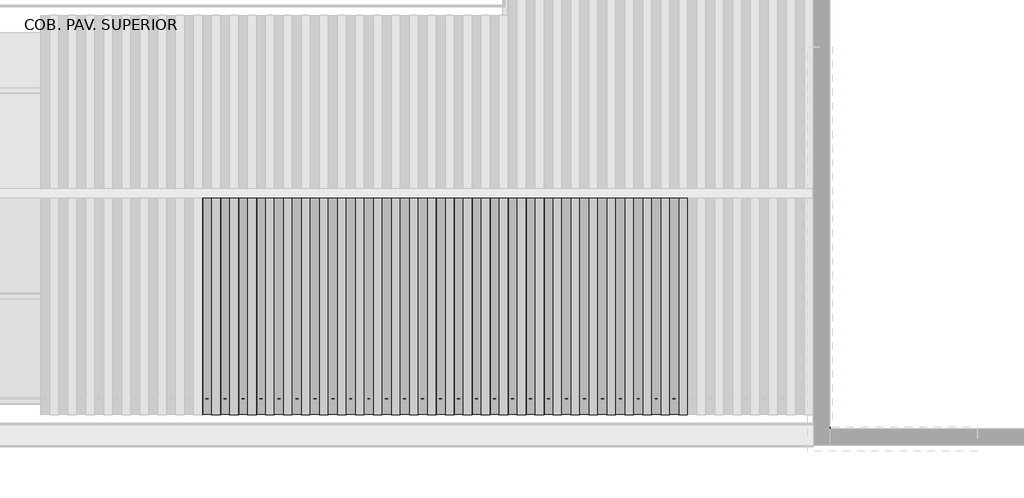
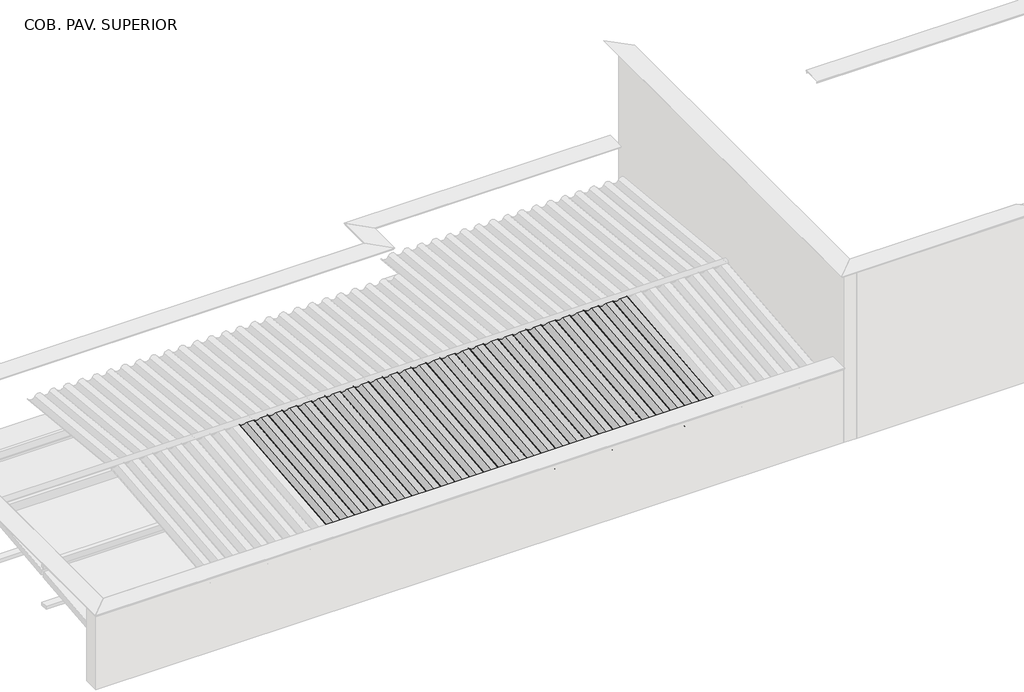
# One storey, part 2 of 7: 35 beams, 8 columns.
"""IFC4 building model written with IfcOpenShell, lengths in millimetres."""

import ifcopenshell
import ifcopenshell.guid

model = None  # the IFC model being written
_history = None  # IfcOwnerHistory: only IFC2X3 demands one
_inside = {}  # id of a spatial element -> (the spatial element, [elements in it])
_under = {}  # id of a project, library or spatial element -> (it, [spatial elements below it])
_declared = {}  # id of a project -> (the project, [libraries it declares])
_typed = {}  # id of a type object -> (the type object, [elements of that type])
_made_of = {}  # id of a material, layer set ... -> (it, [elements and type objects made of it])


def new_model(schema):
    """Start an empty IFC model of exactly this schema.

    Asked for "IFC4X3", IfcOpenShell would pick the latest addendum, in which some entities
    have other attributes; the version numbers below select the first issue.
    IFC2X3 requires an IfcOwnerHistory on every rooted entity: one is made here for all.
    """
    global model, _history
    if schema == "IFC4X3":
        model = ifcopenshell.file(schema_version=(4, 3, 0, 0))
    else:
        model = ifcopenshell.file(schema=schema)
    _inside.clear()
    _under.clear()
    _declared.clear()
    _typed.clear()
    _made_of.clear()
    _history = None
    if model.schema == "IFC2X3":
        org = make("IfcOrganization", Name="unknown")
        user = make(
            "IfcPersonAndOrganization",
            ThePerson=make("IfcPerson", FamilyName="unknown"),
            TheOrganization=org,
        )
        app = make(
            "IfcApplication",
            ApplicationDeveloper=org,
            Version="unknown",
            ApplicationFullName="unknown",
            ApplicationIdentifier="unknown",
        )
        _history = make(
            "IfcOwnerHistory",
            OwningUser=user,
            OwningApplication=app,
            ChangeAction="ADDED",
            CreationDate=0,
        )
    return model


def make(cls, **values):
    """One entity of the class cls with the attributes given. An attribute that is None is left unset."""
    return model.create_entity(
        cls, **{name: value for name, value in values.items() if value is not None}
    )


def rooted(cls, **values):
    """An entity with a GlobalId (a new one), such as an element, a storey or a relation."""
    return make(cls, GlobalId=ifcopenshell.guid.new(), OwnerHistory=_history, **values)


def si_unit(unit_type, name, prefix=None):
    """IfcSIUnit, for example si_unit("LENGTHUNIT", "METRE", prefix="MILLI")."""
    return make("IfcSIUnit", UnitType=unit_type, Prefix=prefix, Name=name)


def assignment(units):
    """IfcUnitAssignment: the units of a project."""
    return None if units is None else make("IfcUnitAssignment", Units=units)


def point(xyz):
    """IfcCartesianPoint."""
    return None if xyz is None else make("IfcCartesianPoint", Coordinates=xyz)


def direction(xyz):
    """IfcDirection."""
    return None if xyz is None else make("IfcDirection", DirectionRatios=xyz)


def frame(location, z_axis=None, x_axis=None):
    """IfcAxis2Placement3D, a coordinate frame: its origin and axes. An axis left out is left unset."""
    return make(
        "IfcAxis2Placement3D",
        Location=point(location),
        Axis=direction(z_axis),
        RefDirection=direction(x_axis),
    )


def frame_2d(location, x_axis=None):
    """IfcAxis2Placement2D, a coordinate frame in the plane: its origin and x axis."""
    return make(
        "IfcAxis2Placement2D", Location=point(location), RefDirection=direction(x_axis)
    )


def origin():
    """The frame at (0, 0, 0) with its axes left unset."""
    return frame((0.0, 0.0, 0.0))


def place(relative_to, where):
    """IfcLocalPlacement: puts the frame where relative to a parent placement (None: the world)."""
    return make(
        "IfcLocalPlacement", PlacementRelTo=relative_to, RelativePlacement=where
    )


def context(
    kind, dimensions, precision=None, world=None, true_north=None, identifier=None
):
    """IfcGeometricRepresentationContext, for example the 3D "Model" context."""
    return make(
        "IfcGeometricRepresentationContext",
        ContextIdentifier=identifier,
        ContextType=kind,
        CoordinateSpaceDimension=dimensions,
        Precision=precision,
        WorldCoordinateSystem=world,
        TrueNorth=true_north,
    )


def project(units=None, contexts=None):
    """IfcProject with its units and contexts."""
    return rooted(
        "IfcProject",
        Name="project",
        RepresentationContexts=contexts,
        UnitsInContext=assignment(units),
    )


def spatial(cls, under=None, at=None, **own):
    """A site, building, storey or space (cls), placed at a placement, below another one or the project."""
    s = rooted(cls, ObjectPlacement=at, **own)
    if under is not None:
        _under.setdefault(under.id(), (under, []))[1].append(s)
    return s


def polyline(points):
    """IfcPolyline through the points."""
    return make("IfcPolyline", Points=[point(p) for p in points])


def circle_curve(where, radius):
    """IfcCircle in the frame where."""
    return make("IfcCircle", Position=where, Radius=radius)


def trimmed(basis, trim1, trim2, sense, master):
    """IfcTrimmedCurve: the piece of a basis curve between two trims."""
    return make(
        "IfcTrimmedCurve",
        BasisCurve=basis,
        Trim1=trim1,
        Trim2=trim2,
        SenseAgreement=sense,
        MasterRepresentation=master,
    )


def segment(curve, same_sense, transition):
    """IfcCompositeCurveSegment."""
    return make(
        "IfcCompositeCurveSegment",
        Transition=transition,
        SameSense=same_sense,
        ParentCurve=curve,
    )


def composite_curve(segments, self_intersect=None):
    """IfcCompositeCurve: segments joined end to end."""
    return make("IfcCompositeCurve", Segments=segments, SelfIntersect=self_intersect)


def outline(outer, holes=None, kind="AREA"):
    """IfcArbitraryClosedProfileDef: a profile drawn as a closed curve; with holes, ...WithVoids."""
    if holes is None:
        return make("IfcArbitraryClosedProfileDef", ProfileType=kind, OuterCurve=outer)
    return make(
        "IfcArbitraryProfileDefWithVoids",
        ProfileType=kind,
        OuterCurve=outer,
        InnerCurves=holes,
    )


def extrude(swept, where, along, depth):
    """IfcExtrudedAreaSolid: the profile swept, set in the frame where, extruded along a direction by depth."""
    return make(
        "IfcExtrudedAreaSolid",
        SweptArea=swept,
        Position=where,
        ExtrudedDirection=direction(along),
        Depth=depth,
    )


def faces_of(points, faces, orient=None, outer=None):
    """IfcFace entities. A face is a list of loops; a loop is a list of indices into points, from 0.

    orient and outer hold one flag for each loop. By default every Orientation is true, the
    first loop of a face is its IfcFaceOuterBound and the others are IfcFaceBound.
    """
    made = []
    for i, loops in enumerate(faces):
        bounds = []
        for j, loop in enumerate(loops):
            is_outer = j == 0 if outer is None else outer[i][j]
            bounds.append(
                make(
                    "IfcFaceOuterBound" if is_outer else "IfcFaceBound",
                    Bound=make("IfcPolyLoop", Polygon=[points[k] for k in loop]),
                    Orientation=True if orient is None else orient[i][j],
                )
            )
        made.append(make("IfcFace", Bounds=bounds))
    return made


def faceted_brep(points, faces, orient=None, outer=None, voids=None):
    """IfcFacetedBrep: a solid bounded by flat faces; with voids (closed shells), ...WithVoids."""
    shared = [point(p) for p in points]
    hull = make("IfcClosedShell", CfsFaces=faces_of(shared, faces, orient, outer))
    if voids is None:
        return make("IfcFacetedBrep", Outer=hull)
    return make(
        "IfcFacetedBrepWithVoids",
        Outer=hull,
        Voids=[
            make(cls, CfsFaces=faces_of(shared, fs, o, b)) for cls, fs, o, b in voids
        ],
    )


def shape(context_of_items, identifier, shape_type, items):
    """IfcShapeRepresentation: the items that make up one representation, for example the "Body"."""
    return make(
        "IfcShapeRepresentation",
        ContextOfItems=context_of_items,
        RepresentationIdentifier=identifier,
        RepresentationType=shape_type,
        Items=items,
    )


def source(mapping_origin, context_of_items, identifier, shape_type, items):
    """IfcRepresentationMap: a shape defined once, which mapped items show again and again."""
    return make(
        "IfcRepresentationMap",
        MappingOrigin=mapping_origin,
        MappedRepresentation=shape(context_of_items, identifier, shape_type, items),
    )


def transform(
    local_origin,
    x_axis=None,
    y_axis=None,
    z_axis=None,
    scale=None,
    scale2=None,
    scale3=None,
    uniform=True,
):
    """IfcCartesianTransformationOperator3D, or its non-uniform kind. x_axis, y_axis, z_axis: its Axis1, 2, 3."""
    if uniform:
        return make(
            "IfcCartesianTransformationOperator3D",
            Axis1=direction(x_axis),
            Axis2=direction(y_axis),
            LocalOrigin=point(local_origin),
            Scale=scale,
            Axis3=direction(z_axis),
        )
    return make(
        "IfcCartesianTransformationOperator3DnonUniform",
        Axis1=direction(x_axis),
        Axis2=direction(y_axis),
        LocalOrigin=point(local_origin),
        Scale=scale,
        Axis3=direction(z_axis),
        Scale2=scale2,
        Scale3=scale3,
    )


def mapped(mapping_source, mapping_target):
    """IfcMappedItem: shows the shape of a source again, moved by a transform."""
    return make(
        "IfcMappedItem", MappingSource=mapping_source, MappingTarget=mapping_target
    )


def made_of(thing, what):
    """Note that an element or type object is made of a material, layer set ...; save() writes the relation."""
    if what is not None:
        _made_of.setdefault(what.id(), (what, []))[1].append(thing)
    return thing


def element(
    cls,
    number,
    at=None,
    inside=None,
    cuts=None,
    type_object=None,
    material=None,
    context=None,
    identifier="Body",
    shape_type=None,
    held_by="IfcProductDefinitionShape",
    body=None,
    shapes=None,
    **own,
):
    """One element of the class cls, such as IfcWall. Its Tag is "e" and its number.

    at: its placement. inside: the storey or other place that contains it. cuts: it is an
    opening in that element (IfcRelVoidsElement). A single representation is given by context,
    identifier, shape_type and body (its items); several are given by shapes. held_by: the class
    of the entity that holds the representations. save() writes the other relations.
    """
    e = rooted(cls, Tag="e%d" % number, ObjectPlacement=at, **own)
    if body is not None:
        shapes = [shape(context, identifier, shape_type, body)]
    if shapes is not None:
        e.Representation = make(held_by, Representations=shapes)
    if inside is not None:
        _inside.setdefault(inside.id(), (inside, []))[1].append(e)
    if cuts is not None:
        rooted(
            "IfcRelVoidsElement", RelatingBuildingElement=cuts, RelatedOpeningElement=e
        )
    if type_object is not None:
        _typed.setdefault(type_object.id(), (type_object, []))[1].append(e)
    return made_of(e, material)


def aggregate(whole, parts):
    """IfcRelAggregates: a whole, such as a stair, and the parts it consists of."""
    return rooted("IfcRelAggregates", RelatingObject=whole, RelatedObjects=parts)


def save(model, path):
    """Write the relations noted so far, then the file.

    IfcRelAggregates (storeys below a building ...), IfcRelContainedInSpatialStructure (elements
    in a storey), IfcRelDefinesByType, IfcRelAssociatesMaterial and IfcRelDeclares: one each for
    every whole, place, type object, material and project.
    """
    for whole, parts in _under.values():
        aggregate(whole, parts)
    for where, things in _inside.values():
        rooted(
            "IfcRelContainedInSpatialStructure",
            RelatedElements=things,
            RelatingStructure=where,
        )
    for kind, things in _typed.values():
        rooted("IfcRelDefinesByType", RelatedObjects=things, RelatingType=kind)
    for what, things in _made_of.values():
        rooted("IfcRelAssociatesMaterial", RelatedObjects=things, RelatingMaterial=what)
    for by, libraries in _declared.values():
        rooted("IfcRelDeclares", RelatingContext=by, RelatedDefinitions=libraries)
    model.write(path)


def column_4db371bd(model_context):
    return source(origin(), model_context, "Body", "SweptSolid", [
        extrude(outline(polyline([(30.0, 80.0), (30.0, -80.0), (-30.0, -80.0), (-30.0, 80.0), (30.0, 80.0)])), frame((0.0, 0.0, 6710.0), z_axis=(0.0, 0.0, 1.0), x_axis=(1.0, 0.0, 0.0)), (0.0, 0.0, 1.0), 660.0),
    ])


def column_e8b88e91(model_context):
    return source(origin(), model_context, "Body", "SweptSolid", [
        extrude(outline(polyline([(30.0, 80.0), (30.0, -80.0), (-30.0, -80.0), (-30.0, 80.0), (30.0, 80.0)])), frame((0.0, 0.0, 6710.0), z_axis=(0.0, 0.0, 1.0), x_axis=(1.0, 0.0, 0.0)), (0.0, 0.0, 1.0), 515.0),
    ])


model = new_model("IFC4")

# Units and contexts
model_context = context("Model", 3, world=origin())
ifc_project = project(units=[si_unit("LENGTHUNIT", "METRE", prefix="MILLI")], contexts=[model_context])

# Site, building, storey
site = spatial("IfcSite", under=ifc_project)
building = spatial("IfcBuilding", under=site)
storey = spatial("IfcBuildingStorey", under=building, Name="COB. PAV. SUPERIOR", Elevation=6650.0)

# Beams
placement = place(None, origin())
element("IfcBeam", 1, ObjectType="Madeira de lei : Berço 6x12cm", at=placement, inside=storey, context=model_context, shape_type="SweptSolid", body=[
    extrude(outline(polyline([(-6679.281307, -9101.268869), (-6679.281307, -9221.268869), (-8679.281307, -9221.268869), (-8679.281307, -9101.268869), (-6679.281307, -9101.268869)])), frame((0.0, 0.0, 6650.0), z_axis=(0.0, 0.0, 1.0), x_axis=(1.0, 0.0, 0.0)), (0.0, 0.0, 1.0), 60.0),
])
element("IfcBeam", 2, ObjectType="Madeira de lei : Berço 6x12cm", at=placement, inside=storey, context=model_context, shape_type="SweptSolid", body=[
    extrude(outline(polyline([(-6679.281307, -10521.818869), (-6679.281307, -10641.818869), (-8679.281307, -10641.818869), (-8679.281307, -10521.818869), (-6679.281307, -10521.818869)])), frame((0.0, 0.0, 6650.0), z_axis=(0.0, 0.0, 1.0), x_axis=(1.0, 0.0, 0.0)), (0.0, 0.0, 1.0), 60.0),
])
element("IfcBeam", 3, ObjectType="Madeira de lei : Berço 6x12cm", at=placement, inside=storey, context=model_context, shape_type="SweptSolid", body=[
    extrude(outline(polyline([(-4679.281307, -9101.268869), (-4679.281307, -9221.268869), (-6679.281307, -9221.268869), (-6679.281307, -9101.268869), (-4679.281307, -9101.268869)])), frame((0.0, 0.0, 6650.0), z_axis=(0.0, 0.0, 1.0), x_axis=(1.0, 0.0, 0.0)), (0.0, 0.0, 1.0), 60.0),
])
element("IfcBeam", 4, ObjectType="Madeira de lei : Berço 6x12cm", at=placement, inside=storey, context=model_context, shape_type="SweptSolid", body=[
    extrude(outline(polyline([(-4679.281307, -10521.818869), (-4679.281307, -10641.818869), (-6679.281307, -10641.818869), (-6679.281307, -10521.818869), (-4679.281307, -10521.818869)])), frame((0.0, 0.0, 6650.0), z_axis=(0.0, 0.0, 1.0), x_axis=(1.0, 0.0, 0.0)), (0.0, 0.0, 1.0), 60.0),
])
element("IfcBeam", 5, ObjectType="Madeira de lei : Berço 6x12cm", at=placement, inside=storey, context=model_context, shape_type="SweptSolid", body=[
    extrude(outline(polyline([(-2679.281307, -9101.268869), (-2679.281307, -9221.268869), (-4679.281307, -9221.268869), (-4679.281307, -9101.268869), (-2679.281307, -9101.268869)])), frame((0.0, 0.0, 6650.0), z_axis=(0.0, 0.0, 1.0), x_axis=(1.0, 0.0, 0.0)), (0.0, 0.0, 1.0), 60.0),
])
element("IfcBeam", 6, ObjectType="Madeira de lei : Berço 6x12cm", at=placement, inside=storey, context=model_context, shape_type="SweptSolid", body=[
    extrude(outline(polyline([(-2679.281307, -10521.818869), (-2679.281307, -10641.818869), (-4679.281307, -10641.818869), (-4679.281307, -10521.818869), (-2679.281307, -10521.818869)])), frame((0.0, 0.0, 6650.0), z_axis=(0.0, 0.0, 1.0), x_axis=(1.0, 0.0, 0.0)), (0.0, 0.0, 1.0), 60.0),
])
element("IfcBeam", 7, ObjectType="Madeira de lei : Berço 6x12cm", at=placement, inside=storey, context=model_context, shape_type="SweptSolid", body=[
    extrude(outline(polyline([(-679.281307, -10521.818869), (-679.281307, -10641.818869), (-2679.281307, -10641.818869), (-2679.281307, -10521.818869), (-679.281307, -10521.818869)])), frame((0.0, 0.0, 6650.0), z_axis=(0.0, 0.0, 1.0), x_axis=(1.0, 0.0, 0.0)), (0.0, 0.0, 1.0), 60.0),
])
element("IfcBeam", 8, ObjectType="Madeira de lei : Berço 6x12cm", at=placement, inside=storey, context=model_context, shape_type="SweptSolid", body=[
    extrude(outline(polyline([(-239.281307, -10521.818869), (-239.281307, -10641.818869), (-679.281307, -10641.818869), (-679.281307, -10521.818869), (-239.281307, -10521.818869)])), frame((0.0, 0.0, 6650.0), z_axis=(0.0, 0.0, 1.0), x_axis=(1.0, 0.0, 0.0)), (0.0, 0.0, 1.0), 60.0),
])
element("IfcBeam", 9, ObjectType="Telha Ondulada : Fibrocimento", at=placement, inside=storey, context=model_context, shape_type="SweptSolid", body=[
    extrude(outline(composite_curve([segment(trimmed(circle_curve(frame_2d((0.0, 66.7939461)), 66.7939461), [point((29.3501489, 6.7939461))], [point((29.3501489, 126.7939461))], True, "CARTESIAN"), True, "CONTINUOUS"), segment(polyline([(29.3501489, 126.7939461), (31.5472154, 131.2853711)]), True, "CONTINUOUS"), segment(trimmed(circle_curve(frame_2d((0.0, 66.7939461)), 71.7939461), [point((31.5472154, 131.2853711))], [point((31.5472154, 2.3025211))], False, "CARTESIAN"), True, "CONTINUOUS"), segment(trimmed(circle_curve(frame_2d((58.7002978, -53.2060539)), 61.7939461), [point((31.5472154, 2.3025211))], [point((31.5472154, -108.7146289))], True, "CARTESIAN"), True, "CONTINUOUS"), segment(polyline([(31.5472154, -108.7146289), (29.3501489, -113.2060539)]), True, "CONTINUOUS"), segment(trimmed(circle_curve(frame_2d((58.7002978, -53.2060539)), 66.7939461), [point((29.3501489, -113.2060539))], [point((29.3501489, 6.7939461))], False, "CARTESIAN"), True, "CONTINUOUS")], self_intersect=False)), frame((-8428.8843743, -10781.9594023, 7394.5315886), z_axis=(0.0, 0.9950371902099894, 0.0995037190209974), x_axis=(0.0, 0.0995037190209974, -0.9950371902099894)), (0.0, 0.0, 1.0), 3017.2295147),
])
element("IfcBeam", 10, ObjectType="Telha Ondulada : Fibrocimento", at=placement, inside=storey, context=model_context, shape_type="SweptSolid", body=[
    extrude(outline(composite_curve([segment(trimmed(circle_curve(frame_2d((0.0, 66.7939461)), 66.7939461), [point((29.3501489, 6.7939461))], [point((29.3501489, 126.7939461))], True, "CARTESIAN"), True, "CONTINUOUS"), segment(polyline([(29.3501489, 126.7939461), (31.5472154, 131.2853711)]), True, "CONTINUOUS"), segment(trimmed(circle_curve(frame_2d((0.0, 66.7939461)), 71.7939461), [point((31.5472154, 131.2853711))], [point((31.5472154, 2.3025211))], False, "CARTESIAN"), True, "CONTINUOUS"), segment(trimmed(circle_curve(frame_2d((58.7002978, -53.2060539)), 61.7939461), [point((31.5472154, 2.3025211))], [point((31.5472154, -108.7146289))], True, "CARTESIAN"), True, "CONTINUOUS"), segment(polyline([(31.5472154, -108.7146289), (29.3501489, -113.2060539)]), True, "CONTINUOUS"), segment(trimmed(circle_curve(frame_2d((58.7002978, -53.2060539)), 66.7939461), [point((29.3501489, -113.2060539))], [point((29.3501489, 6.7939461))], False, "CARTESIAN"), True, "CONTINUOUS")], self_intersect=False)), frame((-8184.3843743, -10781.9594023, 7394.5315886), z_axis=(0.0, 0.9950371902099894, 0.09950371902099736), x_axis=(0.0, 0.09950371902099736, -0.9950371902099894)), (0.0, 0.0, 1.0), 3017.2295147),
])
element("IfcBeam", 11, ObjectType="Telha Ondulada : Fibrocimento", at=placement, inside=storey, context=model_context, shape_type="SweptSolid", body=[
    extrude(outline(composite_curve([segment(trimmed(circle_curve(frame_2d((0.0, 66.7939461)), 66.7939461), [point((29.3501489, 6.7939461))], [point((29.3501489, 126.7939461))], True, "CARTESIAN"), True, "CONTINUOUS"), segment(polyline([(29.3501489, 126.7939461), (31.5472154, 131.2853711)]), True, "CONTINUOUS"), segment(trimmed(circle_curve(frame_2d((0.0, 66.7939461)), 71.7939461), [point((31.5472154, 131.2853711))], [point((31.5472154, 2.3025211))], False, "CARTESIAN"), True, "CONTINUOUS"), segment(trimmed(circle_curve(frame_2d((58.7002978, -53.2060539)), 61.7939461), [point((31.5472154, 2.3025211))], [point((31.5472154, -108.7146289))], True, "CARTESIAN"), True, "CONTINUOUS"), segment(polyline([(31.5472154, -108.7146289), (29.3501489, -113.2060539)]), True, "CONTINUOUS"), segment(trimmed(circle_curve(frame_2d((58.7002978, -53.2060539)), 66.7939461), [point((29.3501489, -113.2060539))], [point((29.3501489, 6.7939461))], False, "CARTESIAN"), True, "CONTINUOUS")], self_intersect=False)), frame((-7939.8843743, -10781.9594023, 7394.5315886), z_axis=(0.0, 0.9950371902099894, 0.09950371902099743), x_axis=(0.0, 0.09950371902099743, -0.9950371902099894)), (0.0, 0.0, 1.0), 3017.2295147),
])
element("IfcBeam", 12, ObjectType="Telha Ondulada : Fibrocimento", at=placement, inside=storey, context=model_context, shape_type="SweptSolid", body=[
    extrude(outline(composite_curve([segment(trimmed(circle_curve(frame_2d((0.0, 66.7939461)), 66.7939461), [point((29.3501489, 6.7939461))], [point((29.3501489, 126.7939461))], True, "CARTESIAN"), True, "CONTINUOUS"), segment(polyline([(29.3501489, 126.7939461), (31.5472154, 131.2853711)]), True, "CONTINUOUS"), segment(trimmed(circle_curve(frame_2d((0.0, 66.7939461)), 71.7939461), [point((31.5472154, 131.2853711))], [point((31.5472154, 2.3025211))], False, "CARTESIAN"), True, "CONTINUOUS"), segment(trimmed(circle_curve(frame_2d((58.7002978, -53.2060539)), 61.7939461), [point((31.5472154, 2.3025211))], [point((31.5472154, -108.7146289))], True, "CARTESIAN"), True, "CONTINUOUS"), segment(polyline([(31.5472154, -108.7146289), (29.3501489, -113.2060539)]), True, "CONTINUOUS"), segment(trimmed(circle_curve(frame_2d((58.7002978, -53.2060539)), 66.7939461), [point((29.3501489, -113.2060539))], [point((29.3501489, 6.7939461))], False, "CARTESIAN"), True, "CONTINUOUS")], self_intersect=False)), frame((-7695.3843743, -10781.9594023, 7394.5315886), z_axis=(0.0, 0.9950371902099894, 0.09950371902099743), x_axis=(0.0, 0.09950371902099743, -0.9950371902099894)), (0.0, 0.0, 1.0), 3017.2295147),
])
element("IfcBeam", 13, ObjectType="Telha Ondulada : Fibrocimento", at=placement, inside=storey, context=model_context, shape_type="SweptSolid", body=[
    extrude(outline(composite_curve([segment(trimmed(circle_curve(frame_2d((0.0, 66.7939461)), 66.7939461), [point((29.3501489, 6.7939461))], [point((29.3501489, 126.7939461))], True, "CARTESIAN"), True, "CONTINUOUS"), segment(polyline([(29.3501489, 126.7939461), (31.5472154, 131.2853711)]), True, "CONTINUOUS"), segment(trimmed(circle_curve(frame_2d((0.0, 66.7939461)), 71.7939461), [point((31.5472154, 131.2853711))], [point((31.5472154, 2.3025211))], False, "CARTESIAN"), True, "CONTINUOUS"), segment(trimmed(circle_curve(frame_2d((58.7002978, -53.2060539)), 61.7939461), [point((31.5472154, 2.3025211))], [point((31.5472154, -108.7146289))], True, "CARTESIAN"), True, "CONTINUOUS"), segment(polyline([(31.5472154, -108.7146289), (29.3501489, -113.2060539)]), True, "CONTINUOUS"), segment(trimmed(circle_curve(frame_2d((58.7002978, -53.2060539)), 66.7939461), [point((29.3501489, -113.2060539))], [point((29.3501489, 6.7939461))], False, "CARTESIAN"), True, "CONTINUOUS")], self_intersect=False)), frame((-7450.8843743, -10781.9594023, 7394.5315886), z_axis=(0.0, 0.9950371902099894, 0.09950371902099743), x_axis=(0.0, 0.09950371902099743, -0.9950371902099894)), (0.0, 0.0, 1.0), 3017.2295147),
])
element("IfcBeam", 14, ObjectType="Telha Ondulada : Fibrocimento", at=placement, inside=storey, context=model_context, shape_type="SweptSolid", body=[
    extrude(outline(composite_curve([segment(trimmed(circle_curve(frame_2d((0.0, 66.7939461)), 66.7939461), [point((29.3501489, 6.7939461))], [point((29.3501489, 126.7939461))], True, "CARTESIAN"), True, "CONTINUOUS"), segment(polyline([(29.3501489, 126.7939461), (31.5472154, 131.2853711)]), True, "CONTINUOUS"), segment(trimmed(circle_curve(frame_2d((0.0, 66.7939461)), 71.7939461), [point((31.5472154, 131.2853711))], [point((31.5472154, 2.3025211))], False, "CARTESIAN"), True, "CONTINUOUS"), segment(trimmed(circle_curve(frame_2d((58.7002978, -53.2060539)), 61.7939461), [point((31.5472154, 2.3025211))], [point((31.5472154, -108.7146289))], True, "CARTESIAN"), True, "CONTINUOUS"), segment(polyline([(31.5472154, -108.7146289), (29.3501489, -113.2060539)]), True, "CONTINUOUS"), segment(trimmed(circle_curve(frame_2d((58.7002978, -53.2060539)), 66.7939461), [point((29.3501489, -113.2060539))], [point((29.3501489, 6.7939461))], False, "CARTESIAN"), True, "CONTINUOUS")], self_intersect=False)), frame((-7206.3843743, -10781.9594023, 7394.5315886), z_axis=(0.0, 0.9950371902099894, 0.0995037190209974), x_axis=(0.0, 0.0995037190209974, -0.9950371902099894)), (0.0, 0.0, 1.0), 3017.2295147),
])
element("IfcBeam", 15, ObjectType="Telha Ondulada : Fibrocimento", at=placement, inside=storey, context=model_context, shape_type="SweptSolid", body=[
    extrude(outline(composite_curve([segment(trimmed(circle_curve(frame_2d((0.0, 66.7939461)), 66.7939461), [point((29.3501489, 6.7939461))], [point((29.3501489, 126.7939461))], True, "CARTESIAN"), True, "CONTINUOUS"), segment(polyline([(29.3501489, 126.7939461), (31.5472154, 131.2853711)]), True, "CONTINUOUS"), segment(trimmed(circle_curve(frame_2d((0.0, 66.7939461)), 71.7939461), [point((31.5472154, 131.2853711))], [point((31.5472154, 2.3025211))], False, "CARTESIAN"), True, "CONTINUOUS"), segment(trimmed(circle_curve(frame_2d((58.7002978, -53.2060539)), 61.7939461), [point((31.5472154, 2.3025211))], [point((31.5472154, -108.7146289))], True, "CARTESIAN"), True, "CONTINUOUS"), segment(polyline([(31.5472154, -108.7146289), (29.3501489, -113.2060539)]), True, "CONTINUOUS"), segment(trimmed(circle_curve(frame_2d((58.7002978, -53.2060539)), 66.7939461), [point((29.3501489, -113.2060539))], [point((29.3501489, 6.7939461))], False, "CARTESIAN"), True, "CONTINUOUS")], self_intersect=False)), frame((-6961.8843743, -10781.9594023, 7394.5315886), z_axis=(0.0, 0.9950371902099894, 0.0995037190209974), x_axis=(0.0, 0.0995037190209974, -0.9950371902099894)), (0.0, 0.0, 1.0), 3017.2295147),
])
element("IfcBeam", 16, ObjectType="Telha Ondulada : Fibrocimento", at=placement, inside=storey, context=model_context, shape_type="SweptSolid", body=[
    extrude(outline(composite_curve([segment(trimmed(circle_curve(frame_2d((0.0, 66.7939461)), 66.7939461), [point((29.3501489, 6.7939461))], [point((29.3501489, 126.7939461))], True, "CARTESIAN"), True, "CONTINUOUS"), segment(polyline([(29.3501489, 126.7939461), (31.5472154, 131.2853711)]), True, "CONTINUOUS"), segment(trimmed(circle_curve(frame_2d((0.0, 66.7939461)), 71.7939461), [point((31.5472154, 131.2853711))], [point((31.5472154, 2.3025211))], False, "CARTESIAN"), True, "CONTINUOUS"), segment(trimmed(circle_curve(frame_2d((58.7002978, -53.2060539)), 61.7939461), [point((31.5472154, 2.3025211))], [point((31.5472154, -108.7146289))], True, "CARTESIAN"), True, "CONTINUOUS"), segment(polyline([(31.5472154, -108.7146289), (29.3501489, -113.2060539)]), True, "CONTINUOUS"), segment(trimmed(circle_curve(frame_2d((58.7002978, -53.2060539)), 66.7939461), [point((29.3501489, -113.2060539))], [point((29.3501489, 6.7939461))], False, "CARTESIAN"), True, "CONTINUOUS")], self_intersect=False)), frame((-6717.3843743, -10781.9594023, 7394.5315886), z_axis=(0.0, 0.9950371902099894, 0.09950371902099743), x_axis=(0.0, 0.09950371902099743, -0.9950371902099894)), (0.0, 0.0, 1.0), 3017.2295147),
])
element("IfcBeam", 17, ObjectType="Telha Ondulada : Fibrocimento", at=placement, inside=storey, context=model_context, shape_type="SweptSolid", body=[
    extrude(outline(composite_curve([segment(trimmed(circle_curve(frame_2d((0.0, 66.7939461)), 66.7939461), [point((29.3501489, 6.7939461))], [point((29.3501489, 126.7939461))], True, "CARTESIAN"), True, "CONTINUOUS"), segment(polyline([(29.3501489, 126.7939461), (31.5472154, 131.2853711)]), True, "CONTINUOUS"), segment(trimmed(circle_curve(frame_2d((0.0, 66.7939461)), 71.7939461), [point((31.5472154, 131.2853711))], [point((31.5472154, 2.3025211))], False, "CARTESIAN"), True, "CONTINUOUS"), segment(trimmed(circle_curve(frame_2d((58.7002978, -53.2060539)), 61.7939461), [point((31.5472154, 2.3025211))], [point((31.5472154, -108.7146289))], True, "CARTESIAN"), True, "CONTINUOUS"), segment(polyline([(31.5472154, -108.7146289), (29.3501489, -113.2060539)]), True, "CONTINUOUS"), segment(trimmed(circle_curve(frame_2d((58.7002978, -53.2060539)), 66.7939461), [point((29.3501489, -113.2060539))], [point((29.3501489, 6.7939461))], False, "CARTESIAN"), True, "CONTINUOUS")], self_intersect=False)), frame((-6472.8843743, -10781.9594023, 7394.5315886), z_axis=(0.0, 0.9950371902099894, 0.09950371902099743), x_axis=(0.0, 0.09950371902099743, -0.9950371902099894)), (0.0, 0.0, 1.0), 3017.2295147),
])
element("IfcBeam", 18, ObjectType="Telha Ondulada : Fibrocimento", at=placement, inside=storey, context=model_context, shape_type="SweptSolid", body=[
    extrude(outline(composite_curve([segment(trimmed(circle_curve(frame_2d((0.0, 66.7939461)), 66.7939461), [point((29.3501489, 6.7939461))], [point((29.3501489, 126.7939461))], True, "CARTESIAN"), True, "CONTINUOUS"), segment(polyline([(29.3501489, 126.7939461), (31.5472154, 131.2853711)]), True, "CONTINUOUS"), segment(trimmed(circle_curve(frame_2d((0.0, 66.7939461)), 71.7939461), [point((31.5472154, 131.2853711))], [point((31.5472154, 2.3025211))], False, "CARTESIAN"), True, "CONTINUOUS"), segment(trimmed(circle_curve(frame_2d((58.7002978, -53.2060539)), 61.7939461), [point((31.5472154, 2.3025211))], [point((31.5472154, -108.7146289))], True, "CARTESIAN"), True, "CONTINUOUS"), segment(polyline([(31.5472154, -108.7146289), (29.3501489, -113.2060539)]), True, "CONTINUOUS"), segment(trimmed(circle_curve(frame_2d((58.7002978, -53.2060539)), 66.7939461), [point((29.3501489, -113.2060539))], [point((29.3501489, 6.7939461))], False, "CARTESIAN"), True, "CONTINUOUS")], self_intersect=False)), frame((-6228.3843743, -10781.9594023, 7394.5315886), z_axis=(0.0, 0.9950371902099894, 0.09950371902099743), x_axis=(0.0, 0.09950371902099743, -0.9950371902099894)), (0.0, 0.0, 1.0), 3017.2295147),
])
element("IfcBeam", 19, ObjectType="Telha Ondulada : Fibrocimento", at=placement, inside=storey, context=model_context, shape_type="SweptSolid", body=[
    extrude(outline(composite_curve([segment(trimmed(circle_curve(frame_2d((0.0, 66.7939461)), 66.7939461), [point((29.3501489, 6.7939461))], [point((29.3501489, 126.7939461))], True, "CARTESIAN"), True, "CONTINUOUS"), segment(polyline([(29.3501489, 126.7939461), (31.5472154, 131.2853711)]), True, "CONTINUOUS"), segment(trimmed(circle_curve(frame_2d((0.0, 66.7939461)), 71.7939461), [point((31.5472154, 131.2853711))], [point((31.5472154, 2.3025211))], False, "CARTESIAN"), True, "CONTINUOUS"), segment(trimmed(circle_curve(frame_2d((58.7002978, -53.2060539)), 61.7939461), [point((31.5472154, 2.3025211))], [point((31.5472154, -108.7146289))], True, "CARTESIAN"), True, "CONTINUOUS"), segment(polyline([(31.5472154, -108.7146289), (29.3501489, -113.2060539)]), True, "CONTINUOUS"), segment(trimmed(circle_curve(frame_2d((58.7002978, -53.2060539)), 66.7939461), [point((29.3501489, -113.2060539))], [point((29.3501489, 6.7939461))], False, "CARTESIAN"), True, "CONTINUOUS")], self_intersect=False)), frame((-5983.8843743, -10781.9594023, 7394.5315886), z_axis=(0.0, 0.9950371902099894, 0.09950371902099743), x_axis=(0.0, 0.09950371902099743, -0.9950371902099894)), (0.0, 0.0, 1.0), 3017.2295147),
])
element("IfcBeam", 20, ObjectType="Telha Ondulada : Fibrocimento", at=placement, inside=storey, context=model_context, shape_type="SweptSolid", body=[
    extrude(outline(composite_curve([segment(trimmed(circle_curve(frame_2d((0.0, 66.7939461)), 66.7939461), [point((29.3501489, 6.7939461))], [point((29.3501489, 126.7939461))], True, "CARTESIAN"), True, "CONTINUOUS"), segment(polyline([(29.3501489, 126.7939461), (31.5472154, 131.2853711)]), True, "CONTINUOUS"), segment(trimmed(circle_curve(frame_2d((0.0, 66.7939461)), 71.7939461), [point((31.5472154, 131.2853711))], [point((31.5472154, 2.3025211))], False, "CARTESIAN"), True, "CONTINUOUS"), segment(trimmed(circle_curve(frame_2d((58.7002978, -53.2060539)), 61.7939461), [point((31.5472154, 2.3025211))], [point((31.5472154, -108.7146289))], True, "CARTESIAN"), True, "CONTINUOUS"), segment(polyline([(31.5472154, -108.7146289), (29.3501489, -113.2060539)]), True, "CONTINUOUS"), segment(trimmed(circle_curve(frame_2d((58.7002978, -53.2060539)), 66.7939461), [point((29.3501489, -113.2060539))], [point((29.3501489, 6.7939461))], False, "CARTESIAN"), True, "CONTINUOUS")], self_intersect=False)), frame((-5739.3843743, -10781.9594023, 7394.5315886), z_axis=(0.0, 0.9950371902099894, 0.0995037190209974), x_axis=(0.0, 0.0995037190209974, -0.9950371902099894)), (0.0, 0.0, 1.0), 3017.2295147),
])
element("IfcBeam", 21, ObjectType="Telha Ondulada : Fibrocimento", at=placement, inside=storey, context=model_context, shape_type="SweptSolid", body=[
    extrude(outline(composite_curve([segment(trimmed(circle_curve(frame_2d((0.0, 66.7939461)), 66.7939461), [point((29.3501489, 6.7939461))], [point((29.3501489, 126.7939461))], True, "CARTESIAN"), True, "CONTINUOUS"), segment(polyline([(29.3501489, 126.7939461), (31.5472154, 131.2853711)]), True, "CONTINUOUS"), segment(trimmed(circle_curve(frame_2d((0.0, 66.7939461)), 71.7939461), [point((31.5472154, 131.2853711))], [point((31.5472154, 2.3025211))], False, "CARTESIAN"), True, "CONTINUOUS"), segment(trimmed(circle_curve(frame_2d((58.7002978, -53.2060539)), 61.7939461), [point((31.5472154, 2.3025211))], [point((31.5472154, -108.7146289))], True, "CARTESIAN"), True, "CONTINUOUS"), segment(polyline([(31.5472154, -108.7146289), (29.3501489, -113.2060539)]), True, "CONTINUOUS"), segment(trimmed(circle_curve(frame_2d((58.7002978, -53.2060539)), 66.7939461), [point((29.3501489, -113.2060539))], [point((29.3501489, 6.7939461))], False, "CARTESIAN"), True, "CONTINUOUS")], self_intersect=False)), frame((-5494.8843743, -10781.9594023, 7394.5315886), z_axis=(0.0, 0.9950371902099894, 0.0995037190209974), x_axis=(0.0, 0.0995037190209974, -0.9950371902099894)), (0.0, 0.0, 1.0), 3017.2295147),
])
element("IfcBeam", 22, ObjectType="Telha Ondulada : Fibrocimento", at=placement, inside=storey, context=model_context, shape_type="SweptSolid", body=[
    extrude(outline(composite_curve([segment(trimmed(circle_curve(frame_2d((0.0, 66.7939461)), 66.7939461), [point((29.3501489, 6.7939461))], [point((29.3501489, 126.7939461))], True, "CARTESIAN"), True, "CONTINUOUS"), segment(polyline([(29.3501489, 126.7939461), (31.5472154, 131.2853711)]), True, "CONTINUOUS"), segment(trimmed(circle_curve(frame_2d((0.0, 66.7939461)), 71.7939461), [point((31.5472154, 131.2853711))], [point((31.5472154, 2.3025211))], False, "CARTESIAN"), True, "CONTINUOUS"), segment(trimmed(circle_curve(frame_2d((58.7002978, -53.2060539)), 61.7939461), [point((31.5472154, 2.3025211))], [point((31.5472154, -108.7146289))], True, "CARTESIAN"), True, "CONTINUOUS"), segment(polyline([(31.5472154, -108.7146289), (29.3501489, -113.2060539)]), True, "CONTINUOUS"), segment(trimmed(circle_curve(frame_2d((58.7002978, -53.2060539)), 66.7939461), [point((29.3501489, -113.2060539))], [point((29.3501489, 6.7939461))], False, "CARTESIAN"), True, "CONTINUOUS")], self_intersect=False)), frame((-5250.3843743, -10781.9594023, 7394.5315886), z_axis=(0.0, 0.9950371902099894, 0.09950371902099736), x_axis=(0.0, 0.09950371902099736, -0.9950371902099894)), (0.0, 0.0, 1.0), 3017.2295147),
])
element("IfcBeam", 23, ObjectType="Telha Ondulada : Fibrocimento", at=placement, inside=storey, context=model_context, shape_type="SweptSolid", body=[
    extrude(outline(composite_curve([segment(trimmed(circle_curve(frame_2d((0.0, 66.7939461)), 66.7939461), [point((29.3501489, 6.7939461))], [point((29.3501489, 126.7939461))], True, "CARTESIAN"), True, "CONTINUOUS"), segment(polyline([(29.3501489, 126.7939461), (31.5472154, 131.2853711)]), True, "CONTINUOUS"), segment(trimmed(circle_curve(frame_2d((0.0, 66.7939461)), 71.7939461), [point((31.5472154, 131.2853711))], [point((31.5472154, 2.3025211))], False, "CARTESIAN"), True, "CONTINUOUS"), segment(trimmed(circle_curve(frame_2d((58.7002978, -53.2060539)), 61.7939461), [point((31.5472154, 2.3025211))], [point((31.5472154, -108.7146289))], True, "CARTESIAN"), True, "CONTINUOUS"), segment(polyline([(31.5472154, -108.7146289), (29.3501489, -113.2060539)]), True, "CONTINUOUS"), segment(trimmed(circle_curve(frame_2d((58.7002978, -53.2060539)), 66.7939461), [point((29.3501489, -113.2060539))], [point((29.3501489, 6.7939461))], False, "CARTESIAN"), True, "CONTINUOUS")], self_intersect=False)), frame((-5005.8843743, -10781.9594023, 7394.5315886), z_axis=(0.0, 0.9950371902099894, 0.09950371902099743), x_axis=(0.0, 0.09950371902099743, -0.9950371902099894)), (0.0, 0.0, 1.0), 3017.2295147),
])
element("IfcBeam", 24, ObjectType="Telha Ondulada : Fibrocimento", at=placement, inside=storey, context=model_context, shape_type="SweptSolid", body=[
    extrude(outline(composite_curve([segment(trimmed(circle_curve(frame_2d((0.0, 66.7939461)), 66.7939461), [point((29.3501489, 6.7939461))], [point((29.3501489, 126.7939461))], True, "CARTESIAN"), True, "CONTINUOUS"), segment(polyline([(29.3501489, 126.7939461), (31.5472154, 131.2853711)]), True, "CONTINUOUS"), segment(trimmed(circle_curve(frame_2d((0.0, 66.7939461)), 71.7939461), [point((31.5472154, 131.2853711))], [point((31.5472154, 2.3025211))], False, "CARTESIAN"), True, "CONTINUOUS"), segment(trimmed(circle_curve(frame_2d((58.7002978, -53.2060539)), 61.7939461), [point((31.5472154, 2.3025211))], [point((31.5472154, -108.7146289))], True, "CARTESIAN"), True, "CONTINUOUS"), segment(polyline([(31.5472154, -108.7146289), (29.3501489, -113.2060539)]), True, "CONTINUOUS"), segment(trimmed(circle_curve(frame_2d((58.7002978, -53.2060539)), 66.7939461), [point((29.3501489, -113.2060539))], [point((29.3501489, 6.7939461))], False, "CARTESIAN"), True, "CONTINUOUS")], self_intersect=False)), frame((-4761.3843743, -10781.9594023, 7394.5315886), z_axis=(0.0, 0.9950371902099894, 0.09950371902099743), x_axis=(0.0, 0.09950371902099743, -0.9950371902099894)), (0.0, 0.0, 1.0), 3017.2295147),
])
element("IfcBeam", 25, ObjectType="Telha Ondulada : Fibrocimento", at=placement, inside=storey, context=model_context, shape_type="SweptSolid", body=[
    extrude(outline(composite_curve([segment(trimmed(circle_curve(frame_2d((0.0, 66.7939461)), 66.7939461), [point((29.3501489, 6.7939461))], [point((29.3501489, 126.7939461))], True, "CARTESIAN"), True, "CONTINUOUS"), segment(polyline([(29.3501489, 126.7939461), (31.5472154, 131.2853711)]), True, "CONTINUOUS"), segment(trimmed(circle_curve(frame_2d((0.0, 66.7939461)), 71.7939461), [point((31.5472154, 131.2853711))], [point((31.5472154, 2.3025211))], False, "CARTESIAN"), True, "CONTINUOUS"), segment(trimmed(circle_curve(frame_2d((58.7002978, -53.2060539)), 61.7939461), [point((31.5472154, 2.3025211))], [point((31.5472154, -108.7146289))], True, "CARTESIAN"), True, "CONTINUOUS"), segment(polyline([(31.5472154, -108.7146289), (29.3501489, -113.2060539)]), True, "CONTINUOUS"), segment(trimmed(circle_curve(frame_2d((58.7002978, -53.2060539)), 66.7939461), [point((29.3501489, -113.2060539))], [point((29.3501489, 6.7939461))], False, "CARTESIAN"), True, "CONTINUOUS")], self_intersect=False)), frame((-4516.8843743, -10781.9594023, 7394.5315886), z_axis=(0.0, 0.9950371902099894, 0.09950371902099743), x_axis=(0.0, 0.09950371902099743, -0.9950371902099894)), (0.0, 0.0, 1.0), 3017.2295147),
])
element("IfcBeam", 26, ObjectType="Telha Ondulada : Fibrocimento", at=placement, inside=storey, context=model_context, shape_type="SweptSolid", body=[
    extrude(outline(composite_curve([segment(trimmed(circle_curve(frame_2d((0.0, 66.7939461)), 66.7939461), [point((29.3501489, 6.7939461))], [point((29.3501489, 126.7939461))], True, "CARTESIAN"), True, "CONTINUOUS"), segment(polyline([(29.3501489, 126.7939461), (31.5472154, 131.2853711)]), True, "CONTINUOUS"), segment(trimmed(circle_curve(frame_2d((0.0, 66.7939461)), 71.7939461), [point((31.5472154, 131.2853711))], [point((31.5472154, 2.3025211))], False, "CARTESIAN"), True, "CONTINUOUS"), segment(trimmed(circle_curve(frame_2d((58.7002978, -53.2060539)), 61.7939461), [point((31.5472154, 2.3025211))], [point((31.5472154, -108.7146289))], True, "CARTESIAN"), True, "CONTINUOUS"), segment(polyline([(31.5472154, -108.7146289), (29.3501489, -113.2060539)]), True, "CONTINUOUS"), segment(trimmed(circle_curve(frame_2d((58.7002978, -53.2060539)), 66.7939461), [point((29.3501489, -113.2060539))], [point((29.3501489, 6.7939461))], False, "CARTESIAN"), True, "CONTINUOUS")], self_intersect=False)), frame((-4272.3843743, -10781.9594023, 7394.5315886), z_axis=(0.0, 0.9950371902099894, 0.0995037190209974), x_axis=(0.0, 0.0995037190209974, -0.9950371902099894)), (0.0, 0.0, 1.0), 3017.2295147),
])
element("IfcBeam", 27, ObjectType="Telha Ondulada : Fibrocimento", at=placement, inside=storey, context=model_context, shape_type="SweptSolid", body=[
    extrude(outline(composite_curve([segment(trimmed(circle_curve(frame_2d((0.0, 66.7939461)), 66.7939461), [point((29.3501489, 6.7939461))], [point((29.3501489, 126.7939461))], True, "CARTESIAN"), True, "CONTINUOUS"), segment(polyline([(29.3501489, 126.7939461), (31.5472154, 131.2853711)]), True, "CONTINUOUS"), segment(trimmed(circle_curve(frame_2d((0.0, 66.7939461)), 71.7939461), [point((31.5472154, 131.2853711))], [point((31.5472154, 2.3025211))], False, "CARTESIAN"), True, "CONTINUOUS"), segment(trimmed(circle_curve(frame_2d((58.7002978, -53.2060539)), 61.7939461), [point((31.5472154, 2.3025211))], [point((31.5472154, -108.7146289))], True, "CARTESIAN"), True, "CONTINUOUS"), segment(polyline([(31.5472154, -108.7146289), (29.3501489, -113.2060539)]), True, "CONTINUOUS"), segment(trimmed(circle_curve(frame_2d((58.7002978, -53.2060539)), 66.7939461), [point((29.3501489, -113.2060539))], [point((29.3501489, 6.7939461))], False, "CARTESIAN"), True, "CONTINUOUS")], self_intersect=False)), frame((-4027.8843743, -10781.9594023, 7394.5315886), z_axis=(0.0, 0.9950371902099894, 0.0995037190209974), x_axis=(0.0, 0.0995037190209974, -0.9950371902099894)), (0.0, 0.0, 1.0), 3017.2295147),
])
element("IfcBeam", 28, ObjectType="Telha Ondulada : Fibrocimento", at=placement, inside=storey, context=model_context, shape_type="SweptSolid", body=[
    extrude(outline(composite_curve([segment(trimmed(circle_curve(frame_2d((0.0, 66.7939461)), 66.7939461), [point((29.3501489, 6.7939461))], [point((29.3501489, 126.7939461))], True, "CARTESIAN"), True, "CONTINUOUS"), segment(polyline([(29.3501489, 126.7939461), (31.5472154, 131.2853711)]), True, "CONTINUOUS"), segment(trimmed(circle_curve(frame_2d((0.0, 66.7939461)), 71.7939461), [point((31.5472154, 131.2853711))], [point((31.5472154, 2.3025211))], False, "CARTESIAN"), True, "CONTINUOUS"), segment(trimmed(circle_curve(frame_2d((58.7002978, -53.2060539)), 61.7939461), [point((31.5472154, 2.3025211))], [point((31.5472154, -108.7146289))], True, "CARTESIAN"), True, "CONTINUOUS"), segment(polyline([(31.5472154, -108.7146289), (29.3501489, -113.2060539)]), True, "CONTINUOUS"), segment(trimmed(circle_curve(frame_2d((58.7002978, -53.2060539)), 66.7939461), [point((29.3501489, -113.2060539))], [point((29.3501489, 6.7939461))], False, "CARTESIAN"), True, "CONTINUOUS")], self_intersect=False)), frame((-3783.3843743, -10781.9594023, 7394.5315886), z_axis=(0.0, 0.9950371902099894, 0.09950371902099743), x_axis=(0.0, 0.09950371902099743, -0.9950371902099894)), (0.0, 0.0, 1.0), 3017.2295147),
])
element("IfcBeam", 29, ObjectType="Telha Ondulada : Fibrocimento", at=placement, inside=storey, context=model_context, shape_type="SweptSolid", body=[
    extrude(outline(composite_curve([segment(trimmed(circle_curve(frame_2d((0.0, 66.7939461)), 66.7939461), [point((29.3501489, 6.7939461))], [point((29.3501489, 126.7939461))], True, "CARTESIAN"), True, "CONTINUOUS"), segment(polyline([(29.3501489, 126.7939461), (31.5472154, 131.2853711)]), True, "CONTINUOUS"), segment(trimmed(circle_curve(frame_2d((0.0, 66.7939461)), 71.7939461), [point((31.5472154, 131.2853711))], [point((31.5472154, 2.3025211))], False, "CARTESIAN"), True, "CONTINUOUS"), segment(trimmed(circle_curve(frame_2d((58.7002978, -53.2060539)), 61.7939461), [point((31.5472154, 2.3025211))], [point((31.5472154, -108.7146289))], True, "CARTESIAN"), True, "CONTINUOUS"), segment(polyline([(31.5472154, -108.7146289), (29.3501489, -113.2060539)]), True, "CONTINUOUS"), segment(trimmed(circle_curve(frame_2d((58.7002978, -53.2060539)), 66.7939461), [point((29.3501489, -113.2060539))], [point((29.3501489, 6.7939461))], False, "CARTESIAN"), True, "CONTINUOUS")], self_intersect=False)), frame((-3538.8843743, -10781.9594023, 7394.5315886), z_axis=(0.0, 0.9950371902099894, 0.09950371902099743), x_axis=(0.0, 0.09950371902099743, -0.9950371902099894)), (0.0, 0.0, 1.0), 3017.2295147),
])
element("IfcBeam", 30, ObjectType="Telha Ondulada : Fibrocimento", at=placement, inside=storey, context=model_context, shape_type="SweptSolid", body=[
    extrude(outline(composite_curve([segment(trimmed(circle_curve(frame_2d((0.0, 66.7939461)), 66.7939461), [point((29.3501489, 6.7939461))], [point((29.3501489, 126.7939461))], True, "CARTESIAN"), True, "CONTINUOUS"), segment(polyline([(29.3501489, 126.7939461), (31.5472154, 131.2853711)]), True, "CONTINUOUS"), segment(trimmed(circle_curve(frame_2d((0.0, 66.7939461)), 71.7939461), [point((31.5472154, 131.2853711))], [point((31.5472154, 2.3025211))], False, "CARTESIAN"), True, "CONTINUOUS"), segment(trimmed(circle_curve(frame_2d((58.7002978, -53.2060539)), 61.7939461), [point((31.5472154, 2.3025211))], [point((31.5472154, -108.7146289))], True, "CARTESIAN"), True, "CONTINUOUS"), segment(polyline([(31.5472154, -108.7146289), (29.3501489, -113.2060539)]), True, "CONTINUOUS"), segment(trimmed(circle_curve(frame_2d((58.7002978, -53.2060539)), 66.7939461), [point((29.3501489, -113.2060539))], [point((29.3501489, 6.7939461))], False, "CARTESIAN"), True, "CONTINUOUS")], self_intersect=False)), frame((-3294.3843743, -10781.9594023, 7394.5315886), z_axis=(0.0, 0.9950371902099894, 0.09950371902099743), x_axis=(0.0, 0.09950371902099743, -0.9950371902099894)), (0.0, 0.0, 1.0), 3017.2295147),
])
element("IfcBeam", 31, ObjectType="Telha Ondulada : Fibrocimento", at=placement, inside=storey, context=model_context, shape_type="SweptSolid", body=[
    extrude(outline(composite_curve([segment(trimmed(circle_curve(frame_2d((0.0, 66.7939461)), 66.7939461), [point((29.3501489, 6.7939461))], [point((29.3501489, 126.7939461))], True, "CARTESIAN"), True, "CONTINUOUS"), segment(polyline([(29.3501489, 126.7939461), (31.5472154, 131.2853711)]), True, "CONTINUOUS"), segment(trimmed(circle_curve(frame_2d((0.0, 66.7939461)), 71.7939461), [point((31.5472154, 131.2853711))], [point((31.5472154, 2.3025211))], False, "CARTESIAN"), True, "CONTINUOUS"), segment(trimmed(circle_curve(frame_2d((58.7002978, -53.2060539)), 61.7939461), [point((31.5472154, 2.3025211))], [point((31.5472154, -108.7146289))], True, "CARTESIAN"), True, "CONTINUOUS"), segment(polyline([(31.5472154, -108.7146289), (29.3501489, -113.2060539)]), True, "CONTINUOUS"), segment(trimmed(circle_curve(frame_2d((58.7002978, -53.2060539)), 66.7939461), [point((29.3501489, -113.2060539))], [point((29.3501489, 6.7939461))], False, "CARTESIAN"), True, "CONTINUOUS")], self_intersect=False)), frame((-3049.8843743, -10781.9594023, 7394.5315886), z_axis=(0.0, 0.9950371902099894, 0.0995037190209974), x_axis=(0.0, 0.0995037190209974, -0.9950371902099894)), (0.0, 0.0, 1.0), 3017.2295147),
])
element("IfcBeam", 32, ObjectType="Telha Ondulada : Fibrocimento", at=placement, inside=storey, context=model_context, shape_type="SweptSolid", body=[
    extrude(outline(composite_curve([segment(trimmed(circle_curve(frame_2d((0.0, 66.7939461)), 66.7939461), [point((29.3501489, 6.7939461))], [point((29.3501489, 126.7939461))], True, "CARTESIAN"), True, "CONTINUOUS"), segment(polyline([(29.3501489, 126.7939461), (31.5472154, 131.2853711)]), True, "CONTINUOUS"), segment(trimmed(circle_curve(frame_2d((0.0, 66.7939461)), 71.7939461), [point((31.5472154, 131.2853711))], [point((31.5472154, 2.3025211))], False, "CARTESIAN"), True, "CONTINUOUS"), segment(trimmed(circle_curve(frame_2d((58.7002978, -53.2060539)), 61.7939461), [point((31.5472154, 2.3025211))], [point((31.5472154, -108.7146289))], True, "CARTESIAN"), True, "CONTINUOUS"), segment(polyline([(31.5472154, -108.7146289), (29.3501489, -113.2060539)]), True, "CONTINUOUS"), segment(trimmed(circle_curve(frame_2d((58.7002978, -53.2060539)), 66.7939461), [point((29.3501489, -113.2060539))], [point((29.3501489, 6.7939461))], False, "CARTESIAN"), True, "CONTINUOUS")], self_intersect=False)), frame((-2805.3843743, -10781.9594023, 7394.5315886), z_axis=(0.0, 0.9950371902099894, 0.09950371902099736), x_axis=(0.0, 0.09950371902099736, -0.9950371902099894)), (0.0, 0.0, 1.0), 3017.2295147),
])
element("IfcBeam", 33, ObjectType="Telha Ondulada : Fibrocimento", at=placement, inside=storey, context=model_context, shape_type="SweptSolid", body=[
    extrude(outline(composite_curve([segment(trimmed(circle_curve(frame_2d((0.0, 66.7939461)), 66.7939461), [point((29.3501489, 6.7939461))], [point((29.3501489, 126.7939461))], True, "CARTESIAN"), True, "CONTINUOUS"), segment(polyline([(29.3501489, 126.7939461), (31.5472154, 131.2853711)]), True, "CONTINUOUS"), segment(trimmed(circle_curve(frame_2d((0.0, 66.7939461)), 71.7939461), [point((31.5472154, 131.2853711))], [point((31.5472154, 2.3025211))], False, "CARTESIAN"), True, "CONTINUOUS"), segment(trimmed(circle_curve(frame_2d((58.7002978, -53.2060539)), 61.7939461), [point((31.5472154, 2.3025211))], [point((31.5472154, -108.7146289))], True, "CARTESIAN"), True, "CONTINUOUS"), segment(polyline([(31.5472154, -108.7146289), (29.3501489, -113.2060539)]), True, "CONTINUOUS"), segment(trimmed(circle_curve(frame_2d((58.7002978, -53.2060539)), 66.7939461), [point((29.3501489, -113.2060539))], [point((29.3501489, 6.7939461))], False, "CARTESIAN"), True, "CONTINUOUS")], self_intersect=False)), frame((-2560.8843743, -10781.9594023, 7394.5315886), z_axis=(0.0, 0.9950371902099894, 0.09950371902099736), x_axis=(0.0, 0.09950371902099736, -0.9950371902099894)), (0.0, 0.0, 1.0), 3017.2295147),
])
element("IfcBeam", 34, ObjectType="Telha Ondulada : Fibrocimento", at=placement, inside=storey, context=model_context, shape_type="SweptSolid", body=[
    extrude(outline(composite_curve([segment(trimmed(circle_curve(frame_2d((0.0, 66.7939461)), 66.7939461), [point((29.3501489, 6.7939461))], [point((29.3501489, 126.7939461))], True, "CARTESIAN"), True, "CONTINUOUS"), segment(polyline([(29.3501489, 126.7939461), (31.5472154, 131.2853711)]), True, "CONTINUOUS"), segment(trimmed(circle_curve(frame_2d((0.0, 66.7939461)), 71.7939461), [point((31.5472154, 131.2853711))], [point((31.5472154, 2.3025211))], False, "CARTESIAN"), True, "CONTINUOUS"), segment(trimmed(circle_curve(frame_2d((58.7002978, -53.2060539)), 61.7939461), [point((31.5472154, 2.3025211))], [point((31.5472154, -108.7146289))], True, "CARTESIAN"), True, "CONTINUOUS"), segment(polyline([(31.5472154, -108.7146289), (29.3501489, -113.2060539)]), True, "CONTINUOUS"), segment(trimmed(circle_curve(frame_2d((58.7002978, -53.2060539)), 66.7939461), [point((29.3501489, -113.2060539))], [point((29.3501489, 6.7939461))], False, "CARTESIAN"), True, "CONTINUOUS")], self_intersect=False)), frame((-2316.3843743, -10781.9594023, 7394.5315886), z_axis=(0.0, 0.9950371902099894, 0.09950371902099743), x_axis=(0.0, 0.09950371902099743, -0.9950371902099894)), (0.0, 0.0, 1.0), 3017.2295147),
])
element("IfcBeam", 35, ObjectType="Telha Ondulada : Fibrocimento", at=placement, inside=storey, context=model_context, shape_type="SweptSolid", body=[
    extrude(outline(composite_curve([segment(trimmed(circle_curve(frame_2d((0.0, 66.7939461)), 66.7939461), [point((29.3501489, 6.7939461))], [point((29.3501489, 126.7939461))], True, "CARTESIAN"), True, "CONTINUOUS"), segment(polyline([(29.3501489, 126.7939461), (31.5472154, 131.2853711)]), True, "CONTINUOUS"), segment(trimmed(circle_curve(frame_2d((0.0, 66.7939461)), 71.7939461), [point((31.5472154, 131.2853711))], [point((31.5472154, 2.3025211))], False, "CARTESIAN"), True, "CONTINUOUS"), segment(trimmed(circle_curve(frame_2d((58.7002978, -53.2060539)), 61.7939461), [point((31.5472154, 2.3025211))], [point((31.5472154, -108.7146289))], True, "CARTESIAN"), True, "CONTINUOUS"), segment(polyline([(31.5472154, -108.7146289), (29.3501489, -113.2060539)]), True, "CONTINUOUS"), segment(trimmed(circle_curve(frame_2d((58.7002978, -53.2060539)), 66.7939461), [point((29.3501489, -113.2060539))], [point((29.3501489, 6.7939461))], False, "CARTESIAN"), True, "CONTINUOUS")], self_intersect=False)), frame((-2071.8843743, -10781.9594023, 7394.5315886), z_axis=(0.0, 0.9950371902099894, 0.09950371902099743), x_axis=(0.0, 0.09950371902099743, -0.9950371902099894)), (0.0, 0.0, 1.0), 3017.2295147),
])

# Columns
column_shape = column_4db371bd(model_context)
element("IfcColumn", 36, ObjectType="Madeira de lei-Coluna : Pontalete 6X16cm", at=placement, inside=storey, context=model_context, shape_type="MappedRepresentation", body=[
    mapped(column_shape, transform((-7679.281307, -9161.268869, 0.0), x_axis=(0.0, 1.0, 0.0), y_axis=(-1.0, 0.0, 0.0), z_axis=(0.0, 0.0, 1.0))),
])
element("IfcColumn", 37, ObjectType="Madeira de lei-Coluna : Pontalete 6X16cm", at=placement, inside=storey, context=model_context, shape_type="MappedRepresentation", body=[
    mapped(column_shape, transform((-5679.281307, -9161.268869, 0.0), x_axis=(0.0, 1.0, 0.0), y_axis=(-1.0, 0.0, 0.0), z_axis=(0.0, 0.0, 1.0))),
])
element("IfcColumn", 38, ObjectType="Madeira de lei-Coluna : Pontalete 6X16cm", at=placement, inside=storey, context=model_context, shape_type="MappedRepresentation", body=[
    mapped(column_shape, transform((-3679.281307, -9161.268869, 0.0), x_axis=(0.0, 1.0, 0.0), y_axis=(-1.0, 0.0, 0.0), z_axis=(0.0, 0.0, 1.0))),
])
column_2_shape = column_e8b88e91(model_context)
element("IfcColumn", 39, ObjectType="Madeira de lei-Coluna : Pontalete 6X16cm", at=placement, inside=storey, context=model_context, shape_type="MappedRepresentation", body=[
    mapped(column_2_shape, transform((-7679.281307, -10581.818869, 0.0), x_axis=(0.0, 1.0, 0.0), y_axis=(-1.0, 0.0, 0.0), z_axis=(0.0, 0.0, 1.0))),
])
element("IfcColumn", 40, ObjectType="Madeira de lei-Coluna : Pontalete 6X16cm", at=placement, inside=storey, context=model_context, shape_type="MappedRepresentation", body=[
    mapped(column_2_shape, transform((-5679.281307, -10581.818869, 0.0), x_axis=(0.0, 1.0, 0.0), y_axis=(-1.0, 0.0, 0.0), z_axis=(0.0, 0.0, 1.0))),
])
element("IfcColumn", 41, ObjectType="Madeira de lei-Coluna : Pontalete 6X16cm", at=placement, inside=storey, context=model_context, shape_type="MappedRepresentation", body=[
    mapped(column_2_shape, transform((-3679.281307, -10581.818869, 0.0), x_axis=(0.0, 1.0, 0.0), y_axis=(-1.0, 0.0, 0.0), z_axis=(0.0, 0.0, 1.0))),
])
element("IfcColumn", 42, ObjectType="Madeira de lei-Coluna : Pontalete 6X16cm", at=placement, inside=storey, context=model_context, shape_type="MappedRepresentation", body=[
    mapped(column_2_shape, transform((-1679.281307, -10581.818869, 0.0), x_axis=(0.0, 1.0, 0.0), y_axis=(-1.0, 0.0, 0.0), z_axis=(0.0, 0.0, 1.0))),
])
element("IfcColumn", 43, ObjectType="TQS - Pilar retangular : 19.0 x 19.0", at=placement, inside=storey, context=model_context, shape_type="Brep", body=[
    faceted_brep([(-202.281307, -10953.5699847, 6650.0), (-12.281307, -10953.5699847, 6650.0), (-12.281307, -11143.5699847, 6650.0), (-202.281307, -11143.5699847, 6650.0), (-202.281307, -10953.5699847, 8750.0), (-62.281307, -10953.5699847, 8750.0), (-12.281307, -10953.5699847, 8750.0), (-12.281307, -10953.5699847, 7250.0), (-12.281307, -10953.5699847, 7050.0), (-202.281307, -10953.5699847, 7050.0), (-202.281307, -10953.5699847, 7250.0), (-202.281307, -10953.5699847, 8300.0), (-12.281307, -11143.5699847, 8750.0), (-12.281307, -11143.5699847, 7250.0), (-202.281307, -11143.5699847, 8750.0), (-202.281307, -11143.5699847, 7250.0)], [[[0, 1, 2, 3]], [[4, 5, 6, 7, 8, 1, 0, 9, 10, 11]], [[6, 12, 13, 2, 1, 8, 7]], [[12, 14, 15, 3, 2, 13]], [[14, 4, 11, 10, 9, 0, 3, 15]], [[4, 14, 12, 6, 5]]]),
])

save(model, "model.ifc")

# Revit data of these elements
# Type "Madeira de lei : Berço 6x12cm"
#   A = 0.02 m²
#   Length [instance default] = 1.524 m
#   b = 0.06 m
#   d = 0.12 m
#   Structural Material [instance default] = none
#   Assembly Code = ""
# Type "Telha Ondulada : Fibrocimento"
#   Description = "TELHA ONDULADA FIBROCIMENTO"
#   Cost = 5
#   Length [instance default] = 1.524 m
#   b = 0.07 m
#   h = 0.16 m
#   Structural Material = .TELHA DE FIBROCIMENTO
#   Assembly Code = ""
# Type "Madeira de lei-Coluna : Pontalete 6X16cm"
#   A = 0.01952 m²
#   b = 0.06 m
#   d = 0.16 m
#   Structural Material [instance default] = none
#   Assembly Code = ""
# Type "TQS - Pilar retangular : 19.0 x 19.0"
#   b = 0.19 m
#   h = 0.19 m
#   Structural Material [instance default] = Concrete - Cast-in-Place Concrete
# Elements 1, 2, 3, 4, 5, 6, 7, 8 (IfcBeam, "Madeira de lei : Berço 6x12cm")
#   Comments = ""
#   Structural Material = .MADEIRAMENTO
#   Phase Created = CC_PE
#   Materials on its faces: ".MADEIRAMENTO"
# Elements 9, 10, 11, 12, 13, 14, 15, 16, 17, 18, 19, 20, 21, 22, 23, 24, 25, 26, 27, 28, 29, 30, 31, 32, 33, 34, 35 (IfcBeam, "Telha Ondulada : Fibrocimento")
#   Phase Created = CC_PE
#   Materials on its faces: ".TELHA DE FIBROCIMENTO"
# Elements 36, 37, 38, 39, 40, 41, 42 (IfcColumn, "Madeira de lei-Coluna : Pontalete 6X16cm")
#   Comments = ""
#   Structural Material = .MADEIRAMENTO
#   Phase Created = CC_PE
#   Materials on its faces: ".MADEIRAMENTO"
# Element 43 (IfcColumn, "TQS - Pilar retangular : 19.0 x 19.0")
#   Uso = "ESTRUTURA"
#   Titulo = "PT2"
#   Chave = "PT2//0"
#   Tipo Elemento = "Pilar"
#   SHA1 = "F43D605D1DA00D757641A848CE7023BEF37C9FDC"
#   Revisão = ""
#   Tipo de carga = ""
#   Divisor de flexao = ""
#   Secao = "R 19/30 90°"
#   Configuracao = ""
#   Angulo (graus) = ""
#   Detalhamento = ""
#   Casos de vento manual = ""
#   Tipo = ""
#   Alcas = ""
#   Furos = ""
#   Pino = ""
#   Distribuicao = ""
#   Solidarizado = ""
#   Solidarizar na montagem = ""
#   Unir com o próximo = ""
#   Grupo pre moldado = ""
#   Verificado = ""
#   Concreto C = ""
#   Taxa de armadura (kgf/m³) = 0
#   Carga (tf/m²) = 0
#   Carga (tf/m) = 0
#   Carga (tf) = 0
#   Altura = 2.10 m
#   Rebaixo = 0.00 m
#   Altura da fundacao = 0.00 m
#   Largura = 0.00 m
#   Distancia a face = 0.00 m
#   Distancia ao eixo = 0.00 m
#   Resultado de Ensaios fck (MPa) = 0
#   Unique TQS ID = -428
#   Principal = yes
#   Nasce = yes
#   Morre = yes
#   Cabeca de Pilar = no
#   Structural Material = Concrete - Cast-in-Place Concrete
#   Phase Created = CC_PE
#   Materials on its faces: "Concrete - Cast-in-Place Concrete"
# Materials
#   ".TELHA DE FIBROCIMENTO": class "CC_TELHADO", colour RGB 77 77 76, transparency 0, Description = "TELHA ONDULADA FIBROCIMENTO", Cost = 0
#   "Concrete - Cast-in-Place Concrete": class "Unassigned", colour RGB 192 192 192, transparency 0
#   ".MADEIRAMENTO": class ".CC_MADEIRAS", colour RGB 212 179 113, transparency 0, Cost = 0
